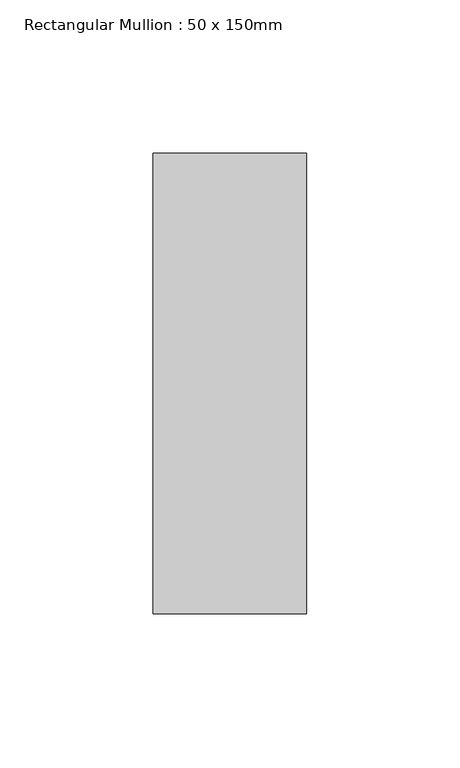
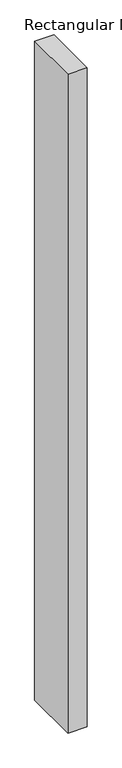
"""IFC4 building model written with IfcOpenShell, lengths in millimetres: member geometry, Rectangular Mullion : 50 x 150mm."""

import ifcopenshell
import ifcopenshell.guid

model = None  # the IFC model being written
_history = None  # IfcOwnerHistory: only IFC2X3 demands one
_inside = {}  # id of a spatial element -> (the spatial element, [elements in it])
_under = {}  # id of a project, library or spatial element -> (it, [spatial elements below it])
_declared = {}  # id of a project -> (the project, [libraries it declares])
_typed = {}  # id of a type object -> (the type object, [elements of that type])
_made_of = {}  # id of a material, layer set ... -> (it, [elements and type objects made of it])


def new_model(schema):
    """Start an empty IFC model of exactly this schema.

    Asked for "IFC4X3", IfcOpenShell would pick the latest addendum, in which some entities
    have other attributes; the version numbers below select the first issue.
    IFC2X3 requires an IfcOwnerHistory on every rooted entity: one is made here for all.
    """
    global model, _history
    if schema == "IFC4X3":
        model = ifcopenshell.file(schema_version=(4, 3, 0, 0))
    else:
        model = ifcopenshell.file(schema=schema)
    _inside.clear()
    _under.clear()
    _declared.clear()
    _typed.clear()
    _made_of.clear()
    _history = None
    if model.schema == "IFC2X3":
        org = make("IfcOrganization", Name="unknown")
        user = make(
            "IfcPersonAndOrganization",
            ThePerson=make("IfcPerson", FamilyName="unknown"),
            TheOrganization=org,
        )
        app = make(
            "IfcApplication",
            ApplicationDeveloper=org,
            Version="unknown",
            ApplicationFullName="unknown",
            ApplicationIdentifier="unknown",
        )
        _history = make(
            "IfcOwnerHistory",
            OwningUser=user,
            OwningApplication=app,
            ChangeAction="ADDED",
            CreationDate=0,
        )
    return model


def make(cls, **values):
    """One entity of the class cls with the attributes given. An attribute that is None is left unset."""
    return model.create_entity(
        cls, **{name: value for name, value in values.items() if value is not None}
    )


def rooted(cls, **values):
    """An entity with a GlobalId (a new one), such as an element, a storey or a relation."""
    return make(cls, GlobalId=ifcopenshell.guid.new(), OwnerHistory=_history, **values)


def si_unit(unit_type, name, prefix=None):
    """IfcSIUnit, for example si_unit("LENGTHUNIT", "METRE", prefix="MILLI")."""
    return make("IfcSIUnit", UnitType=unit_type, Prefix=prefix, Name=name)


def assignment(units):
    """IfcUnitAssignment: the units of a project."""
    return None if units is None else make("IfcUnitAssignment", Units=units)


def point(xyz):
    """IfcCartesianPoint."""
    return None if xyz is None else make("IfcCartesianPoint", Coordinates=xyz)


def direction(xyz):
    """IfcDirection."""
    return None if xyz is None else make("IfcDirection", DirectionRatios=xyz)


def frame(location, z_axis=None, x_axis=None):
    """IfcAxis2Placement3D, a coordinate frame: its origin and axes. An axis left out is left unset."""
    return make(
        "IfcAxis2Placement3D",
        Location=point(location),
        Axis=direction(z_axis),
        RefDirection=direction(x_axis),
    )


def origin():
    """The frame at (0, 0, 0) with its axes left unset."""
    return frame((0.0, 0.0, 0.0))


def place(relative_to, where):
    """IfcLocalPlacement: puts the frame where relative to a parent placement (None: the world)."""
    return make(
        "IfcLocalPlacement", PlacementRelTo=relative_to, RelativePlacement=where
    )


def context(
    kind, dimensions, precision=None, world=None, true_north=None, identifier=None
):
    """IfcGeometricRepresentationContext, for example the 3D "Model" context."""
    return make(
        "IfcGeometricRepresentationContext",
        ContextIdentifier=identifier,
        ContextType=kind,
        CoordinateSpaceDimension=dimensions,
        Precision=precision,
        WorldCoordinateSystem=world,
        TrueNorth=true_north,
    )


def project(units=None, contexts=None):
    """IfcProject with its units and contexts."""
    return rooted(
        "IfcProject",
        Name="project",
        RepresentationContexts=contexts,
        UnitsInContext=assignment(units),
    )


def spatial(cls, under=None, at=None, **own):
    """A site, building, storey or space (cls), placed at a placement, below another one or the project."""
    s = rooted(cls, ObjectPlacement=at, **own)
    if under is not None:
        _under.setdefault(under.id(), (under, []))[1].append(s)
    return s


def polyline(points):
    """IfcPolyline through the points."""
    return make("IfcPolyline", Points=[point(p) for p in points])


def outline(outer, holes=None, kind="AREA"):
    """IfcArbitraryClosedProfileDef: a profile drawn as a closed curve; with holes, ...WithVoids."""
    if holes is None:
        return make("IfcArbitraryClosedProfileDef", ProfileType=kind, OuterCurve=outer)
    return make(
        "IfcArbitraryProfileDefWithVoids",
        ProfileType=kind,
        OuterCurve=outer,
        InnerCurves=holes,
    )


def extrude(swept, where, along, depth):
    """IfcExtrudedAreaSolid: the profile swept, set in the frame where, extruded along a direction by depth."""
    return make(
        "IfcExtrudedAreaSolid",
        SweptArea=swept,
        Position=where,
        ExtrudedDirection=direction(along),
        Depth=depth,
    )


def shape(context_of_items, identifier, shape_type, items):
    """IfcShapeRepresentation: the items that make up one representation, for example the "Body"."""
    return make(
        "IfcShapeRepresentation",
        ContextOfItems=context_of_items,
        RepresentationIdentifier=identifier,
        RepresentationType=shape_type,
        Items=items,
    )


def source(mapping_origin, context_of_items, identifier, shape_type, items):
    """IfcRepresentationMap: a shape defined once, which mapped items show again and again."""
    return make(
        "IfcRepresentationMap",
        MappingOrigin=mapping_origin,
        MappedRepresentation=shape(context_of_items, identifier, shape_type, items),
    )


def transform(
    local_origin,
    x_axis=None,
    y_axis=None,
    z_axis=None,
    scale=None,
    scale2=None,
    scale3=None,
    uniform=True,
):
    """IfcCartesianTransformationOperator3D, or its non-uniform kind. x_axis, y_axis, z_axis: its Axis1, 2, 3."""
    if uniform:
        return make(
            "IfcCartesianTransformationOperator3D",
            Axis1=direction(x_axis),
            Axis2=direction(y_axis),
            LocalOrigin=point(local_origin),
            Scale=scale,
            Axis3=direction(z_axis),
        )
    return make(
        "IfcCartesianTransformationOperator3DnonUniform",
        Axis1=direction(x_axis),
        Axis2=direction(y_axis),
        LocalOrigin=point(local_origin),
        Scale=scale,
        Axis3=direction(z_axis),
        Scale2=scale2,
        Scale3=scale3,
    )


def mapped(mapping_source, mapping_target):
    """IfcMappedItem: shows the shape of a source again, moved by a transform."""
    return make(
        "IfcMappedItem", MappingSource=mapping_source, MappingTarget=mapping_target
    )


def made_of(thing, what):
    """Note that an element or type object is made of a material, layer set ...; save() writes the relation."""
    if what is not None:
        _made_of.setdefault(what.id(), (what, []))[1].append(thing)
    return thing


def element(
    cls,
    number,
    at=None,
    inside=None,
    cuts=None,
    type_object=None,
    material=None,
    context=None,
    identifier="Body",
    shape_type=None,
    held_by="IfcProductDefinitionShape",
    body=None,
    shapes=None,
    **own,
):
    """One element of the class cls, such as IfcWall. Its Tag is "e" and its number.

    at: its placement. inside: the storey or other place that contains it. cuts: it is an
    opening in that element (IfcRelVoidsElement). A single representation is given by context,
    identifier, shape_type and body (its items); several are given by shapes. held_by: the class
    of the entity that holds the representations. save() writes the other relations.
    """
    e = rooted(cls, Tag="e%d" % number, ObjectPlacement=at, **own)
    if body is not None:
        shapes = [shape(context, identifier, shape_type, body)]
    if shapes is not None:
        e.Representation = make(held_by, Representations=shapes)
    if inside is not None:
        _inside.setdefault(inside.id(), (inside, []))[1].append(e)
    if cuts is not None:
        rooted(
            "IfcRelVoidsElement", RelatingBuildingElement=cuts, RelatedOpeningElement=e
        )
    if type_object is not None:
        _typed.setdefault(type_object.id(), (type_object, []))[1].append(e)
    return made_of(e, material)


def aggregate(whole, parts):
    """IfcRelAggregates: a whole, such as a stair, and the parts it consists of."""
    return rooted("IfcRelAggregates", RelatingObject=whole, RelatedObjects=parts)


def save(model, path):
    """Write the relations noted so far, then the file.

    IfcRelAggregates (storeys below a building ...), IfcRelContainedInSpatialStructure (elements
    in a storey), IfcRelDefinesByType, IfcRelAssociatesMaterial and IfcRelDeclares: one each for
    every whole, place, type object, material and project.
    """
    for whole, parts in _under.values():
        aggregate(whole, parts)
    for where, things in _inside.values():
        rooted(
            "IfcRelContainedInSpatialStructure",
            RelatedElements=things,
            RelatingStructure=where,
        )
    for kind, things in _typed.values():
        rooted("IfcRelDefinesByType", RelatedObjects=things, RelatingType=kind)
    for what, things in _made_of.values():
        rooted("IfcRelAssociatesMaterial", RelatedObjects=things, RelatingMaterial=what)
    for by, libraries in _declared.values():
        rooted("IfcRelDeclares", RelatingContext=by, RelatedDefinitions=libraries)
    model.write(path)


def rectangular_mullion_50_x_150mm_4329fe64(model_context):
    return source(origin(), model_context, "Body", "SweptSolid", [
        extrude(outline(polyline([(25.0, 75.0), (25.0, -75.0), (-25.0, -75.0), (-25.0, 75.0), (25.0, 75.0)])), frame((0.0, 0.0, -1813.8888891), z_axis=(0.0, 0.0, 1.0), x_axis=(1.0, 0.0, 0.0)), (0.0, 0.0, 1.0), 1813.8888891),
    ])


if __name__ == "__main__":
    model = new_model("IFC4")
    model_context = context("Model", 3, world=origin())
    ifc_project = project(units=[si_unit("LENGTHUNIT", "METRE", prefix="MILLI")], contexts=[model_context])
    site = spatial("IfcSite", under=ifc_project)
    building = spatial("IfcBuilding", under=site)
    placement = place(None, origin())
    rectangular_mullion_50_x_150mm_shape = rectangular_mullion_50_x_150mm_4329fe64(model_context)
    element("IfcMember", 1, ObjectType="Rectangular Mullion : 50 x 150mm", at=placement, inside=building, context=model_context, shape_type="MappedRepresentation", body=[
        mapped(rectangular_mullion_50_x_150mm_shape, transform((0.0, 0.0, 0.0), x_axis=(1.0, 0.0, 0.0), y_axis=(0.0, 1.0, 0.0), z_axis=(0.0, 0.0, 1.0))),
    ])
    save(model, "model.ifc")

# Revit data of these elements
# Type "Rectangular Mullion : 50 x 150mm"
#   built-in parameter 1007304 = 0.492126 (stored number, unit not read)
#   built-in parameter 1007301 = 0.082021 (stored number, unit not read)
#   built-in parameter 1007300 = 0.082021 (stored number, unit not read)
# Element 1 (IfcMember, "Rectangular Mullion : 50 x 150mm")
#   Materials on its faces: "Metal - Aluminium"
# Materials
#   "Metal - Aluminium": class "Metal", colour RGB 247 247 247, transparency 0
